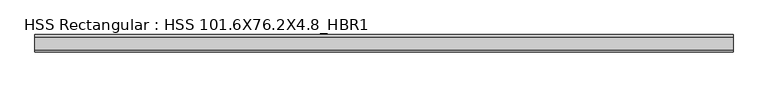
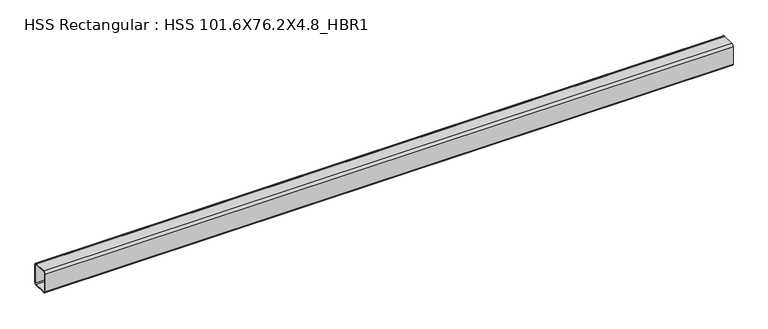
"""IFC4 building model written with IfcOpenShell, lengths in millimetres: beam geometry, HSS Rectangular : HSS 101.6X76.2X4.8_HBR1."""

import ifcopenshell
import ifcopenshell.guid

model = None  # the IFC model being written
_history = None  # IfcOwnerHistory: only IFC2X3 demands one
_inside = {}  # id of a spatial element -> (the spatial element, [elements in it])
_under = {}  # id of a project, library or spatial element -> (it, [spatial elements below it])
_declared = {}  # id of a project -> (the project, [libraries it declares])
_typed = {}  # id of a type object -> (the type object, [elements of that type])
_made_of = {}  # id of a material, layer set ... -> (it, [elements and type objects made of it])


def new_model(schema):
    """Start an empty IFC model of exactly this schema.

    Asked for "IFC4X3", IfcOpenShell would pick the latest addendum, in which some entities
    have other attributes; the version numbers below select the first issue.
    IFC2X3 requires an IfcOwnerHistory on every rooted entity: one is made here for all.
    """
    global model, _history
    if schema == "IFC4X3":
        model = ifcopenshell.file(schema_version=(4, 3, 0, 0))
    else:
        model = ifcopenshell.file(schema=schema)
    _inside.clear()
    _under.clear()
    _declared.clear()
    _typed.clear()
    _made_of.clear()
    _history = None
    if model.schema == "IFC2X3":
        org = make("IfcOrganization", Name="unknown")
        user = make(
            "IfcPersonAndOrganization",
            ThePerson=make("IfcPerson", FamilyName="unknown"),
            TheOrganization=org,
        )
        app = make(
            "IfcApplication",
            ApplicationDeveloper=org,
            Version="unknown",
            ApplicationFullName="unknown",
            ApplicationIdentifier="unknown",
        )
        _history = make(
            "IfcOwnerHistory",
            OwningUser=user,
            OwningApplication=app,
            ChangeAction="ADDED",
            CreationDate=0,
        )
    return model


def make(cls, **values):
    """One entity of the class cls with the attributes given. An attribute that is None is left unset."""
    return model.create_entity(
        cls, **{name: value for name, value in values.items() if value is not None}
    )


def rooted(cls, **values):
    """An entity with a GlobalId (a new one), such as an element, a storey or a relation."""
    return make(cls, GlobalId=ifcopenshell.guid.new(), OwnerHistory=_history, **values)


def si_unit(unit_type, name, prefix=None):
    """IfcSIUnit, for example si_unit("LENGTHUNIT", "METRE", prefix="MILLI")."""
    return make("IfcSIUnit", UnitType=unit_type, Prefix=prefix, Name=name)


def assignment(units):
    """IfcUnitAssignment: the units of a project."""
    return None if units is None else make("IfcUnitAssignment", Units=units)


def point(xyz):
    """IfcCartesianPoint."""
    return None if xyz is None else make("IfcCartesianPoint", Coordinates=xyz)


def direction(xyz):
    """IfcDirection."""
    return None if xyz is None else make("IfcDirection", DirectionRatios=xyz)


def frame(location, z_axis=None, x_axis=None):
    """IfcAxis2Placement3D, a coordinate frame: its origin and axes. An axis left out is left unset."""
    return make(
        "IfcAxis2Placement3D",
        Location=point(location),
        Axis=direction(z_axis),
        RefDirection=direction(x_axis),
    )


def frame_2d(location, x_axis=None):
    """IfcAxis2Placement2D, a coordinate frame in the plane: its origin and x axis."""
    return make(
        "IfcAxis2Placement2D", Location=point(location), RefDirection=direction(x_axis)
    )


def origin():
    """The frame at (0, 0, 0) with its axes left unset."""
    return frame((0.0, 0.0, 0.0))


def place(relative_to, where):
    """IfcLocalPlacement: puts the frame where relative to a parent placement (None: the world)."""
    return make(
        "IfcLocalPlacement", PlacementRelTo=relative_to, RelativePlacement=where
    )


def context(
    kind, dimensions, precision=None, world=None, true_north=None, identifier=None
):
    """IfcGeometricRepresentationContext, for example the 3D "Model" context."""
    return make(
        "IfcGeometricRepresentationContext",
        ContextIdentifier=identifier,
        ContextType=kind,
        CoordinateSpaceDimension=dimensions,
        Precision=precision,
        WorldCoordinateSystem=world,
        TrueNorth=true_north,
    )


def project(units=None, contexts=None):
    """IfcProject with its units and contexts."""
    return rooted(
        "IfcProject",
        Name="project",
        RepresentationContexts=contexts,
        UnitsInContext=assignment(units),
    )


def spatial(cls, under=None, at=None, **own):
    """A site, building, storey or space (cls), placed at a placement, below another one or the project."""
    s = rooted(cls, ObjectPlacement=at, **own)
    if under is not None:
        _under.setdefault(under.id(), (under, []))[1].append(s)
    return s


def polyline(points):
    """IfcPolyline through the points."""
    return make("IfcPolyline", Points=[point(p) for p in points])


def circle_curve(where, radius):
    """IfcCircle in the frame where."""
    return make("IfcCircle", Position=where, Radius=radius)


def trimmed(basis, trim1, trim2, sense, master):
    """IfcTrimmedCurve: the piece of a basis curve between two trims."""
    return make(
        "IfcTrimmedCurve",
        BasisCurve=basis,
        Trim1=trim1,
        Trim2=trim2,
        SenseAgreement=sense,
        MasterRepresentation=master,
    )


def segment(curve, same_sense, transition):
    """IfcCompositeCurveSegment."""
    return make(
        "IfcCompositeCurveSegment",
        Transition=transition,
        SameSense=same_sense,
        ParentCurve=curve,
    )


def composite_curve(segments, self_intersect=None):
    """IfcCompositeCurve: segments joined end to end."""
    return make("IfcCompositeCurve", Segments=segments, SelfIntersect=self_intersect)


def outline(outer, holes=None, kind="AREA"):
    """IfcArbitraryClosedProfileDef: a profile drawn as a closed curve; with holes, ...WithVoids."""
    if holes is None:
        return make("IfcArbitraryClosedProfileDef", ProfileType=kind, OuterCurve=outer)
    return make(
        "IfcArbitraryProfileDefWithVoids",
        ProfileType=kind,
        OuterCurve=outer,
        InnerCurves=holes,
    )


def extrude(swept, where, along, depth):
    """IfcExtrudedAreaSolid: the profile swept, set in the frame where, extruded along a direction by depth."""
    return make(
        "IfcExtrudedAreaSolid",
        SweptArea=swept,
        Position=where,
        ExtrudedDirection=direction(along),
        Depth=depth,
    )


def shape(context_of_items, identifier, shape_type, items):
    """IfcShapeRepresentation: the items that make up one representation, for example the "Body"."""
    return make(
        "IfcShapeRepresentation",
        ContextOfItems=context_of_items,
        RepresentationIdentifier=identifier,
        RepresentationType=shape_type,
        Items=items,
    )


def source(mapping_origin, context_of_items, identifier, shape_type, items):
    """IfcRepresentationMap: a shape defined once, which mapped items show again and again."""
    return make(
        "IfcRepresentationMap",
        MappingOrigin=mapping_origin,
        MappedRepresentation=shape(context_of_items, identifier, shape_type, items),
    )


def transform(
    local_origin,
    x_axis=None,
    y_axis=None,
    z_axis=None,
    scale=None,
    scale2=None,
    scale3=None,
    uniform=True,
):
    """IfcCartesianTransformationOperator3D, or its non-uniform kind. x_axis, y_axis, z_axis: its Axis1, 2, 3."""
    if uniform:
        return make(
            "IfcCartesianTransformationOperator3D",
            Axis1=direction(x_axis),
            Axis2=direction(y_axis),
            LocalOrigin=point(local_origin),
            Scale=scale,
            Axis3=direction(z_axis),
        )
    return make(
        "IfcCartesianTransformationOperator3DnonUniform",
        Axis1=direction(x_axis),
        Axis2=direction(y_axis),
        LocalOrigin=point(local_origin),
        Scale=scale,
        Axis3=direction(z_axis),
        Scale2=scale2,
        Scale3=scale3,
    )


def mapped(mapping_source, mapping_target):
    """IfcMappedItem: shows the shape of a source again, moved by a transform."""
    return make(
        "IfcMappedItem", MappingSource=mapping_source, MappingTarget=mapping_target
    )


def made_of(thing, what):
    """Note that an element or type object is made of a material, layer set ...; save() writes the relation."""
    if what is not None:
        _made_of.setdefault(what.id(), (what, []))[1].append(thing)
    return thing


def element(
    cls,
    number,
    at=None,
    inside=None,
    cuts=None,
    type_object=None,
    material=None,
    context=None,
    identifier="Body",
    shape_type=None,
    held_by="IfcProductDefinitionShape",
    body=None,
    shapes=None,
    **own,
):
    """One element of the class cls, such as IfcWall. Its Tag is "e" and its number.

    at: its placement. inside: the storey or other place that contains it. cuts: it is an
    opening in that element (IfcRelVoidsElement). A single representation is given by context,
    identifier, shape_type and body (its items); several are given by shapes. held_by: the class
    of the entity that holds the representations. save() writes the other relations.
    """
    e = rooted(cls, Tag="e%d" % number, ObjectPlacement=at, **own)
    if body is not None:
        shapes = [shape(context, identifier, shape_type, body)]
    if shapes is not None:
        e.Representation = make(held_by, Representations=shapes)
    if inside is not None:
        _inside.setdefault(inside.id(), (inside, []))[1].append(e)
    if cuts is not None:
        rooted(
            "IfcRelVoidsElement", RelatingBuildingElement=cuts, RelatedOpeningElement=e
        )
    if type_object is not None:
        _typed.setdefault(type_object.id(), (type_object, []))[1].append(e)
    return made_of(e, material)


def aggregate(whole, parts):
    """IfcRelAggregates: a whole, such as a stair, and the parts it consists of."""
    return rooted("IfcRelAggregates", RelatingObject=whole, RelatedObjects=parts)


def save(model, path):
    """Write the relations noted so far, then the file.

    IfcRelAggregates (storeys below a building ...), IfcRelContainedInSpatialStructure (elements
    in a storey), IfcRelDefinesByType, IfcRelAssociatesMaterial and IfcRelDeclares: one each for
    every whole, place, type object, material and project.
    """
    for whole, parts in _under.values():
        aggregate(whole, parts)
    for where, things in _inside.values():
        rooted(
            "IfcRelContainedInSpatialStructure",
            RelatedElements=things,
            RelatingStructure=where,
        )
    for kind, things in _typed.values():
        rooted("IfcRelDefinesByType", RelatedObjects=things, RelatingType=kind)
    for what, things in _made_of.values():
        rooted("IfcRelAssociatesMaterial", RelatedObjects=things, RelatingMaterial=what)
    for by, libraries in _declared.values():
        rooted("IfcRelDeclares", RelatingContext=by, RelatedDefinitions=libraries)
    model.write(path)


def hss_rectangular_hss_101_6x76_2x4_8_hbr1_0fbde055(model_context):
    return source(origin(), model_context, "Body", "SweptSolid", [
        extrude(outline(composite_curve([segment(polyline([(38.1, 41.275), (38.1, -41.275)]), True, "CONTINUOUS"), segment(trimmed(circle_curve(frame_2d((28.575, -41.275)), 9.525), [point((38.1, -41.275))], [point((28.575, -50.8))], False, "CARTESIAN"), True, "CONTINUOUS"), segment(polyline([(28.575, -50.8), (-28.575, -50.8)]), True, "CONTINUOUS"), segment(trimmed(circle_curve(frame_2d((-28.575, -41.275)), 9.525), [point((-28.575, -50.8))], [point((-38.1, -41.275))], False, "CARTESIAN"), True, "CONTINUOUS"), segment(polyline([(-38.1, -41.275), (-38.1, 41.275)]), True, "CONTINUOUS"), segment(trimmed(circle_curve(frame_2d((-28.575, 41.275)), 9.525), [point((-38.1, 41.275))], [point((-28.575, 50.8))], False, "CARTESIAN"), True, "CONTINUOUS"), segment(polyline([(-28.575, 50.8), (28.575, 50.8)]), True, "CONTINUOUS"), segment(trimmed(circle_curve(frame_2d((28.575, 41.275)), 9.525), [point((28.575, 50.8))], [point((38.1, 41.275))], False, "CARTESIAN"), True, "CONTINUOUS")], self_intersect=False), holes=[composite_curve([segment(trimmed(circle_curve(frame_2d((-28.575, 41.275)), 4.7625), [point((-28.575, 46.0375))], [point((-33.3375, 41.275))], True, "CARTESIAN"), True, "CONTINUOUS"), segment(polyline([(-33.3375, 41.275), (-33.3375, -41.275)]), True, "CONTINUOUS"), segment(trimmed(circle_curve(frame_2d((-28.575, -41.275)), 4.7625), [point((-33.3375, -41.275))], [point((-28.575, -46.0375))], True, "CARTESIAN"), True, "CONTINUOUS"), segment(polyline([(-28.575, -46.0375), (28.575, -46.0375)]), True, "CONTINUOUS"), segment(trimmed(circle_curve(frame_2d((28.575, -41.275)), 4.7625), [point((28.575, -46.0375))], [point((33.3375, -41.275))], True, "CARTESIAN"), True, "CONTINUOUS"), segment(polyline([(33.3375, -41.275), (33.3375, 41.275)]), True, "CONTINUOUS"), segment(trimmed(circle_curve(frame_2d((28.575, 41.275)), 4.7625), [point((33.3375, 41.275))], [point((28.575, 46.0375))], True, "CARTESIAN"), True, "CONTINUOUS"), segment(polyline([(28.575, 46.0375), (-28.575, 46.0375)]), True, "CONTINUOUS")], self_intersect=False)]), frame((-1493.2658211, 0.0, 0.0), z_axis=(1.0, 0.0, 0.0), x_axis=(0.0, 1.0, 0.0)), (0.0, 0.0, 1.0), 3066.9601738),
    ])


if __name__ == "__main__":
    model = new_model("IFC4")
    model_context = context("Model", 3, world=origin())
    ifc_project = project(units=[si_unit("LENGTHUNIT", "METRE", prefix="MILLI")], contexts=[model_context])
    site = spatial("IfcSite", under=ifc_project)
    building = spatial("IfcBuilding", under=site)
    placement = place(None, origin())
    hss_rectangular_hss_101_6x76_2x4_8_hbr1_shape = hss_rectangular_hss_101_6x76_2x4_8_hbr1_0fbde055(model_context)
    element("IfcBeam", 1, ObjectType="HSS Rectangular : HSS 101.6X76.2X4.8_HBR1", at=placement, inside=building, context=model_context, shape_type="MappedRepresentation", body=[
        mapped(hss_rectangular_hss_101_6x76_2x4_8_hbr1_shape, transform((0.0, 0.0, 0.0), x_axis=(1.0, 0.0, 0.0), y_axis=(0.0, 1.0, 0.0), z_axis=(0.0, 0.0, 1.0))),
    ])
    save(model, "model.ifc")

# Revit data of these elements
# Type "HSS Rectangular : HSS 101.6X76.2X4.8_HBR1"
#   Section Name Key = "HSS 4X3X3/16"
#   Assembly Code = "B10"
#   Width = 7.62 cm
#   Wall Nominal Thickness = 0.4763 cm
#   Wall Design Thickness = 0.442 cm
#   Torsional Moment of Inertia = 260.561 cm⁴
#   Torsional Modulus = 61.2876 cm³
#   Section Area = 14.4516 cm²
#   Plastic Modulus weak axis = 40.3122 cm³
#   Plastic Modulus strong axis = 49.1612 cm³
#   Perimeter = 0.881482 m²/m
#   Outer Fillet = 0.9525 cm
#   Nominal Weight = 12.1285 kgf/m
#   Moment of Inertia weak axis = 131.529 cm⁴
#   Moment of Inertia strong axis = 205.202 cm⁴
#   Inner Fillet = 0.4763 cm
#   Height = 10.16 cm
#   Elastic Modulus weak axis = 34.4128 cm³
#   Elastic Modulus strong axis = 40.476 cm³
#   Centroid Vertical = 5.08 cm
#   Centroid Horizontal = 3.81 cm
#   Length [instance default] = 1524 mm
#   Structural Material [instance default] = Steel ASTM A500, Grade B, Rectangular and Square
#   Principal Axes Angle = 0
# Element 1 (IfcBeam, "HSS Rectangular : HSS 101.6X76.2X4.8_HBR1")
#   Structural Material = Steel ASTM A992
#   Materials on its faces: "Steel ASTM A992"
# Materials
#   "Steel ASTM A500, Grade B, Rectangular and Square": class "Metal", colour RGB 199 199 199, transparency 0, Description = "Carbon steel", Cost = 0
#   "Steel ASTM A992": class "Metal", colour RGB 199 199 199, transparency 0, Description = "Structural steel 50ksi", Cost = 0
